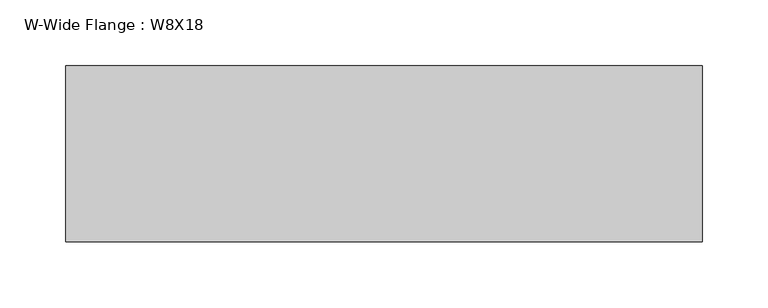
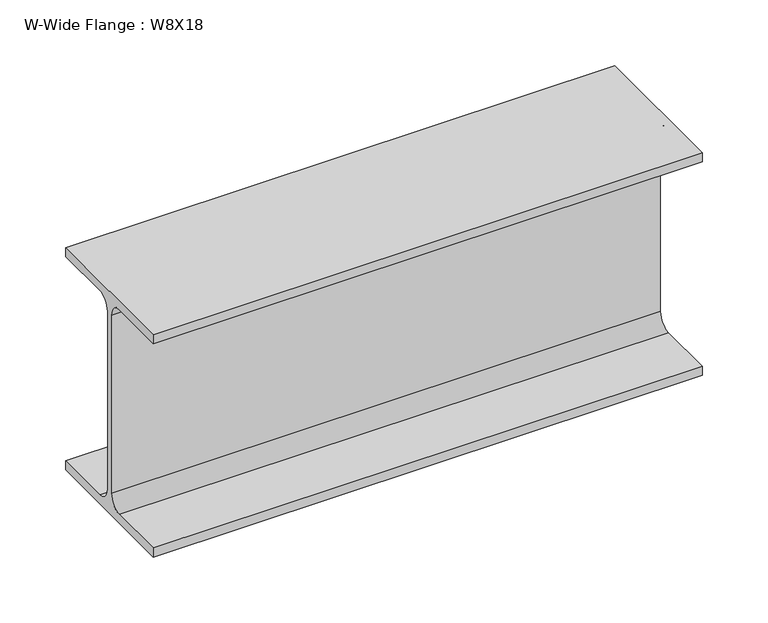
"""IFC4 building model written with IfcOpenShell, lengths in millimetres: beam geometry, W-Wide Flange : W8X18."""

import ifcopenshell
import ifcopenshell.guid

model = None  # the IFC model being written
_history = None  # IfcOwnerHistory: only IFC2X3 demands one
_inside = {}  # id of a spatial element -> (the spatial element, [elements in it])
_under = {}  # id of a project, library or spatial element -> (it, [spatial elements below it])
_declared = {}  # id of a project -> (the project, [libraries it declares])
_typed = {}  # id of a type object -> (the type object, [elements of that type])
_made_of = {}  # id of a material, layer set ... -> (it, [elements and type objects made of it])


def new_model(schema):
    """Start an empty IFC model of exactly this schema.

    Asked for "IFC4X3", IfcOpenShell would pick the latest addendum, in which some entities
    have other attributes; the version numbers below select the first issue.
    IFC2X3 requires an IfcOwnerHistory on every rooted entity: one is made here for all.
    """
    global model, _history
    if schema == "IFC4X3":
        model = ifcopenshell.file(schema_version=(4, 3, 0, 0))
    else:
        model = ifcopenshell.file(schema=schema)
    _inside.clear()
    _under.clear()
    _declared.clear()
    _typed.clear()
    _made_of.clear()
    _history = None
    if model.schema == "IFC2X3":
        org = make("IfcOrganization", Name="unknown")
        user = make(
            "IfcPersonAndOrganization",
            ThePerson=make("IfcPerson", FamilyName="unknown"),
            TheOrganization=org,
        )
        app = make(
            "IfcApplication",
            ApplicationDeveloper=org,
            Version="unknown",
            ApplicationFullName="unknown",
            ApplicationIdentifier="unknown",
        )
        _history = make(
            "IfcOwnerHistory",
            OwningUser=user,
            OwningApplication=app,
            ChangeAction="ADDED",
            CreationDate=0,
        )
    return model


def make(cls, **values):
    """One entity of the class cls with the attributes given. An attribute that is None is left unset."""
    return model.create_entity(
        cls, **{name: value for name, value in values.items() if value is not None}
    )


def rooted(cls, **values):
    """An entity with a GlobalId (a new one), such as an element, a storey or a relation."""
    return make(cls, GlobalId=ifcopenshell.guid.new(), OwnerHistory=_history, **values)


def si_unit(unit_type, name, prefix=None):
    """IfcSIUnit, for example si_unit("LENGTHUNIT", "METRE", prefix="MILLI")."""
    return make("IfcSIUnit", UnitType=unit_type, Prefix=prefix, Name=name)


def assignment(units):
    """IfcUnitAssignment: the units of a project."""
    return None if units is None else make("IfcUnitAssignment", Units=units)


def point(xyz):
    """IfcCartesianPoint."""
    return None if xyz is None else make("IfcCartesianPoint", Coordinates=xyz)


def direction(xyz):
    """IfcDirection."""
    return None if xyz is None else make("IfcDirection", DirectionRatios=xyz)


def frame(location, z_axis=None, x_axis=None):
    """IfcAxis2Placement3D, a coordinate frame: its origin and axes. An axis left out is left unset."""
    return make(
        "IfcAxis2Placement3D",
        Location=point(location),
        Axis=direction(z_axis),
        RefDirection=direction(x_axis),
    )


def frame_2d(location, x_axis=None):
    """IfcAxis2Placement2D, a coordinate frame in the plane: its origin and x axis."""
    return make(
        "IfcAxis2Placement2D", Location=point(location), RefDirection=direction(x_axis)
    )


def origin():
    """The frame at (0, 0, 0) with its axes left unset."""
    return frame((0.0, 0.0, 0.0))


def place(relative_to, where):
    """IfcLocalPlacement: puts the frame where relative to a parent placement (None: the world)."""
    return make(
        "IfcLocalPlacement", PlacementRelTo=relative_to, RelativePlacement=where
    )


def context(
    kind, dimensions, precision=None, world=None, true_north=None, identifier=None
):
    """IfcGeometricRepresentationContext, for example the 3D "Model" context."""
    return make(
        "IfcGeometricRepresentationContext",
        ContextIdentifier=identifier,
        ContextType=kind,
        CoordinateSpaceDimension=dimensions,
        Precision=precision,
        WorldCoordinateSystem=world,
        TrueNorth=true_north,
    )


def project(units=None, contexts=None):
    """IfcProject with its units and contexts."""
    return rooted(
        "IfcProject",
        Name="project",
        RepresentationContexts=contexts,
        UnitsInContext=assignment(units),
    )


def spatial(cls, under=None, at=None, **own):
    """A site, building, storey or space (cls), placed at a placement, below another one or the project."""
    s = rooted(cls, ObjectPlacement=at, **own)
    if under is not None:
        _under.setdefault(under.id(), (under, []))[1].append(s)
    return s


def polyline(points):
    """IfcPolyline through the points."""
    return make("IfcPolyline", Points=[point(p) for p in points])


def circle_curve(where, radius):
    """IfcCircle in the frame where."""
    return make("IfcCircle", Position=where, Radius=radius)


def trimmed(basis, trim1, trim2, sense, master):
    """IfcTrimmedCurve: the piece of a basis curve between two trims."""
    return make(
        "IfcTrimmedCurve",
        BasisCurve=basis,
        Trim1=trim1,
        Trim2=trim2,
        SenseAgreement=sense,
        MasterRepresentation=master,
    )


def segment(curve, same_sense, transition):
    """IfcCompositeCurveSegment."""
    return make(
        "IfcCompositeCurveSegment",
        Transition=transition,
        SameSense=same_sense,
        ParentCurve=curve,
    )


def composite_curve(segments, self_intersect=None):
    """IfcCompositeCurve: segments joined end to end."""
    return make("IfcCompositeCurve", Segments=segments, SelfIntersect=self_intersect)


def outline(outer, holes=None, kind="AREA"):
    """IfcArbitraryClosedProfileDef: a profile drawn as a closed curve; with holes, ...WithVoids."""
    if holes is None:
        return make("IfcArbitraryClosedProfileDef", ProfileType=kind, OuterCurve=outer)
    return make(
        "IfcArbitraryProfileDefWithVoids",
        ProfileType=kind,
        OuterCurve=outer,
        InnerCurves=holes,
    )


def extrude(swept, where, along, depth):
    """IfcExtrudedAreaSolid: the profile swept, set in the frame where, extruded along a direction by depth."""
    return make(
        "IfcExtrudedAreaSolid",
        SweptArea=swept,
        Position=where,
        ExtrudedDirection=direction(along),
        Depth=depth,
    )


def shape(context_of_items, identifier, shape_type, items):
    """IfcShapeRepresentation: the items that make up one representation, for example the "Body"."""
    return make(
        "IfcShapeRepresentation",
        ContextOfItems=context_of_items,
        RepresentationIdentifier=identifier,
        RepresentationType=shape_type,
        Items=items,
    )


def source(mapping_origin, context_of_items, identifier, shape_type, items):
    """IfcRepresentationMap: a shape defined once, which mapped items show again and again."""
    return make(
        "IfcRepresentationMap",
        MappingOrigin=mapping_origin,
        MappedRepresentation=shape(context_of_items, identifier, shape_type, items),
    )


def transform(
    local_origin,
    x_axis=None,
    y_axis=None,
    z_axis=None,
    scale=None,
    scale2=None,
    scale3=None,
    uniform=True,
):
    """IfcCartesianTransformationOperator3D, or its non-uniform kind. x_axis, y_axis, z_axis: its Axis1, 2, 3."""
    if uniform:
        return make(
            "IfcCartesianTransformationOperator3D",
            Axis1=direction(x_axis),
            Axis2=direction(y_axis),
            LocalOrigin=point(local_origin),
            Scale=scale,
            Axis3=direction(z_axis),
        )
    return make(
        "IfcCartesianTransformationOperator3DnonUniform",
        Axis1=direction(x_axis),
        Axis2=direction(y_axis),
        LocalOrigin=point(local_origin),
        Scale=scale,
        Axis3=direction(z_axis),
        Scale2=scale2,
        Scale3=scale3,
    )


def mapped(mapping_source, mapping_target):
    """IfcMappedItem: shows the shape of a source again, moved by a transform."""
    return make(
        "IfcMappedItem", MappingSource=mapping_source, MappingTarget=mapping_target
    )


def made_of(thing, what):
    """Note that an element or type object is made of a material, layer set ...; save() writes the relation."""
    if what is not None:
        _made_of.setdefault(what.id(), (what, []))[1].append(thing)
    return thing


def element(
    cls,
    number,
    at=None,
    inside=None,
    cuts=None,
    type_object=None,
    material=None,
    context=None,
    identifier="Body",
    shape_type=None,
    held_by="IfcProductDefinitionShape",
    body=None,
    shapes=None,
    **own,
):
    """One element of the class cls, such as IfcWall. Its Tag is "e" and its number.

    at: its placement. inside: the storey or other place that contains it. cuts: it is an
    opening in that element (IfcRelVoidsElement). A single representation is given by context,
    identifier, shape_type and body (its items); several are given by shapes. held_by: the class
    of the entity that holds the representations. save() writes the other relations.
    """
    e = rooted(cls, Tag="e%d" % number, ObjectPlacement=at, **own)
    if body is not None:
        shapes = [shape(context, identifier, shape_type, body)]
    if shapes is not None:
        e.Representation = make(held_by, Representations=shapes)
    if inside is not None:
        _inside.setdefault(inside.id(), (inside, []))[1].append(e)
    if cuts is not None:
        rooted(
            "IfcRelVoidsElement", RelatingBuildingElement=cuts, RelatedOpeningElement=e
        )
    if type_object is not None:
        _typed.setdefault(type_object.id(), (type_object, []))[1].append(e)
    return made_of(e, material)


def aggregate(whole, parts):
    """IfcRelAggregates: a whole, such as a stair, and the parts it consists of."""
    return rooted("IfcRelAggregates", RelatingObject=whole, RelatedObjects=parts)


def save(model, path):
    """Write the relations noted so far, then the file.

    IfcRelAggregates (storeys below a building ...), IfcRelContainedInSpatialStructure (elements
    in a storey), IfcRelDefinesByType, IfcRelAssociatesMaterial and IfcRelDeclares: one each for
    every whole, place, type object, material and project.
    """
    for whole, parts in _under.values():
        aggregate(whole, parts)
    for where, things in _inside.values():
        rooted(
            "IfcRelContainedInSpatialStructure",
            RelatedElements=things,
            RelatingStructure=where,
        )
    for kind, things in _typed.values():
        rooted("IfcRelDefinesByType", RelatedObjects=things, RelatingType=kind)
    for what, things in _made_of.values():
        rooted("IfcRelAssociatesMaterial", RelatedObjects=things, RelatingMaterial=what)
    for by, libraries in _declared.values():
        rooted("IfcRelDeclares", RelatingContext=by, RelatedDefinitions=libraries)
    model.write(path)


def w_wide_flange_w8x18_4e8d9058(model_context):
    return source(origin(), model_context, "Body", "SweptSolid", [
        extrude(outline(composite_curve([segment(polyline([(66.675, -94.996), (66.675, -103.378), (-66.675, -103.378), (-66.675, -94.996), (-15.1765, -94.996)]), True, "CONTINUOUS"), segment(trimmed(circle_curve(frame_2d((-15.1765, -82.7405)), 12.2555), [point((-15.1765, -94.996))], [point((-2.921, -82.7405))], True, "CARTESIAN"), True, "CONTINUOUS"), segment(polyline([(-2.921, -82.7405), (-2.921, 82.7405)]), True, "CONTINUOUS"), segment(trimmed(circle_curve(frame_2d((-15.1765, 82.7405)), 12.2555), [point((-2.921, 82.7405))], [point((-15.1765, 94.996))], True, "CARTESIAN"), True, "CONTINUOUS"), segment(polyline([(-15.1765, 94.996), (-66.675, 94.996), (-66.675, 103.378), (66.675, 103.378), (66.675, 94.996), (15.1765, 94.996)]), True, "CONTINUOUS"), segment(trimmed(circle_curve(frame_2d((15.1765, 82.7405)), 12.2555), [point((15.1765, 94.996))], [point((2.921, 82.7405))], True, "CARTESIAN"), True, "CONTINUOUS"), segment(polyline([(2.921, 82.7405), (2.921, -82.7405)]), True, "CONTINUOUS"), segment(trimmed(circle_curve(frame_2d((15.1765, -82.7405)), 12.2555), [point((2.921, -82.7405))], [point((15.1765, -94.996))], True, "CARTESIAN"), True, "CONTINUOUS"), segment(polyline([(15.1765, -94.996), (66.675, -94.996)]), True, "CONTINUOUS")], self_intersect=False)), frame((-241.3, 0.0, 0.0), z_axis=(1.0, 0.0, 0.0), x_axis=(0.0, 1.0, 0.0)), (0.0, 0.0, 1.0), 482.6),
    ])


if __name__ == "__main__":
    model = new_model("IFC4")
    model_context = context("Model", 3, world=origin())
    ifc_project = project(units=[si_unit("LENGTHUNIT", "METRE", prefix="MILLI")], contexts=[model_context])
    site = spatial("IfcSite", under=ifc_project)
    building = spatial("IfcBuilding", under=site)
    placement = place(None, origin())
    w_wide_flange_w8x18_shape = w_wide_flange_w8x18_4e8d9058(model_context)
    element("IfcBeam", 1, ObjectType="W-Wide Flange : W8X18", at=placement, inside=building, context=model_context, shape_type="MappedRepresentation", body=[
        mapped(w_wide_flange_w8x18_shape, transform((0.0, 0.0, 0.0), x_axis=(1.0, 0.0, 0.0), y_axis=(0.0, 1.0, 0.0), z_axis=(0.0, 0.0, 1.0))),
    ])
    save(model, "model.ifc")

# Revit data of these elements
# Type "W-Wide Flange : W8X18"
#   Assembly Code = "B10"
#   W = 18
#   Length [instance default] = 5' - 0"
#   bf = 0' - 5 1/4"
#   d = 0' - 8.14"
#   k = 0' - 0 13/16"
#   k2 = 0' - 0.4825"
#   tf = 0' - 0.33"
#   tw = 0' - 0.23"
#   A = 0.0365278 SF
#   Structural Material [instance default] = _STRUCTURAL STEEL (SEE STRUCT. DWGS)
# Element 1 (IfcBeam, "W-Wide Flange : W8X18")
#   Materials on its faces: "_STRUCTURAL STEEL (SEE STRUCT. DWGS)"
# Materials
#   "_STRUCTURAL STEEL (SEE STRUCT. DWGS)": class "Metal", colour RGB 199 199 199, transparency 0, Description = "Structural steel 50ksi", Cost = 0
